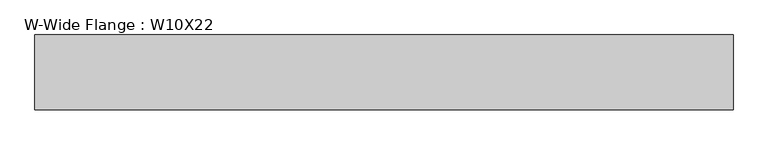
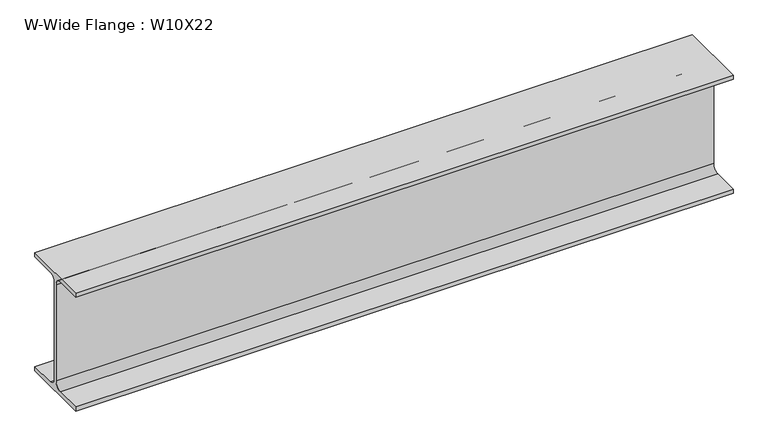
"""IFC4 building model written with IfcOpenShell, lengths in millimetres: beam geometry, W-Wide Flange : W10X22."""

from ifc_helpers import new_model, si_unit, point, frame, frame_2d, origin, place, context, project, spatial, polyline, circle_curve, trimmed, segment, composite_curve, outline, extrude, source, transform, mapped, element, save


def w_wide_flange_w10x22_3ad2fafd(model_context):
    return source(origin(), model_context, "Body", "SweptSolid", [
        extrude(outline(composite_curve([segment(polyline([(73.025, -120.396), (73.025, -129.54), (-73.025, -129.54), (-73.025, -120.396), (-17.7165, -120.396)]), True, "CONTINUOUS"), segment(trimmed(circle_curve(frame_2d((-17.7165, -105.7275)), 14.6685), [point((-17.7165, -120.396))], [point((-3.048, -105.7275))], True, "CARTESIAN"), True, "CONTINUOUS"), segment(polyline([(-3.048, -105.7275), (-3.048, 105.7275)]), True, "CONTINUOUS"), segment(trimmed(circle_curve(frame_2d((-17.7165, 105.7275)), 14.6685), [point((-3.048, 105.7275))], [point((-17.7165, 120.396))], True, "CARTESIAN"), True, "CONTINUOUS"), segment(polyline([(-17.7165, 120.396), (-73.025, 120.396), (-73.025, 129.54), (73.025, 129.54), (73.025, 120.396), (17.7165, 120.396)]), True, "CONTINUOUS"), segment(trimmed(circle_curve(frame_2d((17.7165, 105.7275)), 14.6685), [point((17.7165, 120.396))], [point((3.048, 105.7275))], True, "CARTESIAN"), True, "CONTINUOUS"), segment(polyline([(3.048, 105.7275), (3.048, -105.7275)]), True, "CONTINUOUS"), segment(trimmed(circle_curve(frame_2d((17.7165, -105.7275)), 14.6685), [point((3.048, -105.7275))], [point((17.7165, -120.396))], True, "CARTESIAN"), True, "CONTINUOUS"), segment(polyline([(17.7165, -120.396), (73.025, -120.396)]), True, "CONTINUOUS")], self_intersect=False)), frame((-1328.8645, 0.0, 0.0), z_axis=(1.0, 0.0, 0.0), x_axis=(0.0, 1.0, 0.0)), (0.0, 0.0, 1.0), 1365.25),
    ])


if __name__ == "__main__":
    model = new_model("IFC4")
    model_context = context("Model", 3, world=origin())
    ifc_project = project(units=[si_unit("LENGTHUNIT", "METRE", prefix="MILLI")], contexts=[model_context])
    site = spatial("IfcSite", under=ifc_project)
    building = spatial("IfcBuilding", under=site)
    placement = place(None, origin())
    w_wide_flange_w10x22_shape = w_wide_flange_w10x22_3ad2fafd(model_context)
    element("IfcBeam", 1, ObjectType="W-Wide Flange : W10X22", at=placement, inside=building, context=model_context, shape_type="MappedRepresentation", body=[
        mapped(w_wide_flange_w10x22_shape, transform((0.0, 0.0, 0.0), x_axis=(1.0, 0.0, 0.0), y_axis=(0.0, 1.0, 0.0), z_axis=(0.0, 0.0, 1.0))),
    ])
    save(model, "model.ifc")

# Revit data of these elements
# Type "W-Wide Flange : W10X22"
#   Assembly Code = "B10"
#   W = 22
#   Length [instance default] = 5' - 0"
#   bf = 0' - 5 3/4"
#   d = 0' - 10.2"
#   k = 0' - 0 15/16"
#   k2 = 0' - 0.5775"
#   tf = 0' - 0.36"
#   tw = 0' - 0.24"
#   A = 0.0450694 SF
#   Structural Material [instance default] = _STRUCTURAL STEEL (SEE STRUCT. DWGS)
# Element 1 (IfcBeam, "W-Wide Flange : W10X22")
#   Materials on its faces: "_STRUCTURAL STEEL (SEE STRUCT. DWGS)"
# Materials
#   "_STRUCTURAL STEEL (SEE STRUCT. DWGS)": class "Metal", colour RGB 199 199 199, transparency 0, Description = "Structural steel 50ksi", Cost = 0
